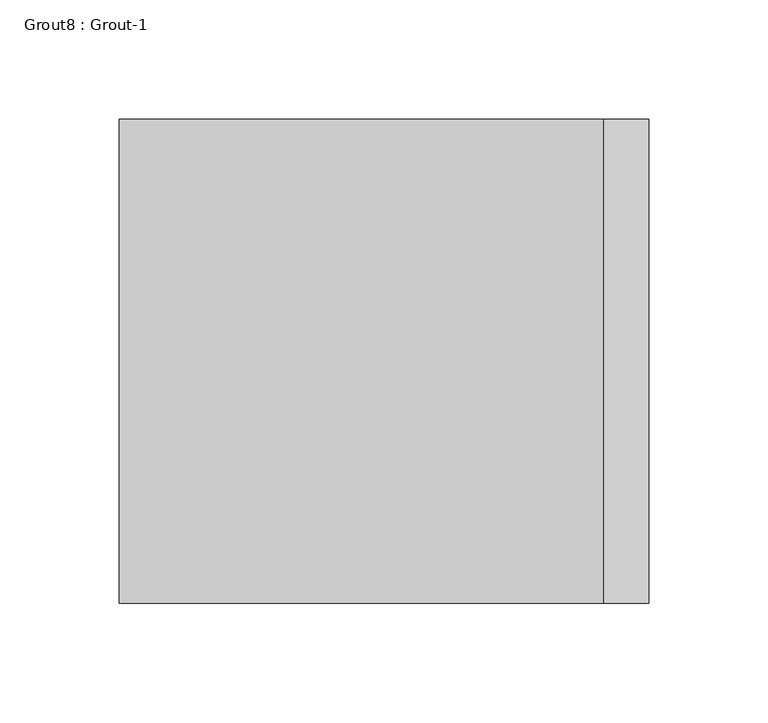
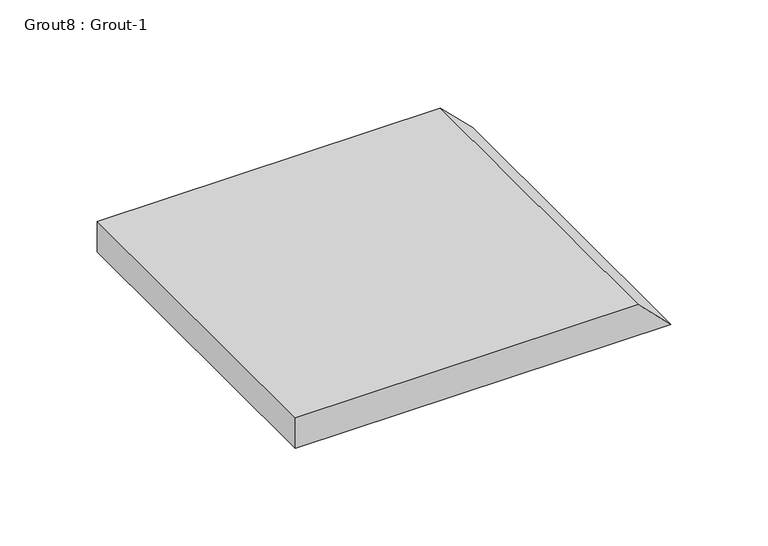
"""IFC4 building model written with IfcOpenShell, lengths in millimetres: proxy geometry, Grout8 : Grout-1."""

from ifc_helpers import new_model, si_unit, frame, origin, place, context, project, spatial, polyline, outline, extrude, source, transform, mapped, element, save


def grout8_grout_1_13d29c56(model_context):
    return source(origin(), model_context, "Body", "SweptSolid", [
        extrude(outline(polyline([(19.05, 587569.0934739), (19.05, 587365.8934739), (0.0, 587365.8934739), (0.0, 587588.1434739), (19.05, 587569.0934739)])), frame((0.0, -536468.3913841, 0.0), z_axis=(0.0, 1.0, 0.0), x_axis=(0.0, 0.0, 1.0)), (0.0, 0.0, 1.0), 203.2),
    ])


if __name__ == "__main__":
    model = new_model("IFC4")
    model_context = context("Model", 3, world=origin())
    ifc_project = project(units=[si_unit("LENGTHUNIT", "METRE", prefix="MILLI")], contexts=[model_context])
    site = spatial("IfcSite", under=ifc_project)
    building = spatial("IfcBuilding", under=site)
    placement = place(None, origin())
    grout8_grout_1_shape = grout8_grout_1_13d29c56(model_context)
    element("IfcBuildingElementProxy", 1, Name="Grout8 : Grout-1", ObjectType="Grout8 : Grout-1", at=placement, inside=building, context=model_context, shape_type="MappedRepresentation", body=[
        mapped(grout8_grout_1_shape, transform((0.0, 0.0, 0.0), x_axis=(1.0, 0.0, 0.0), y_axis=(0.0, 1.0, 0.0), z_axis=(0.0, 0.0, 1.0))),
    ])
    save(model, "model.ifc")

# Revit data of these elements
# Element 1 (IfcBuildingElementProxy, "Grout8 : Grout-1")
#   Materials on its faces: "3/4\" NON SHRINK GROUT"
# Materials
#   "3/4\" NON SHRINK GROUT": class "Generic", colour RGB 145 145 143, transparency 0, Cost = 0
